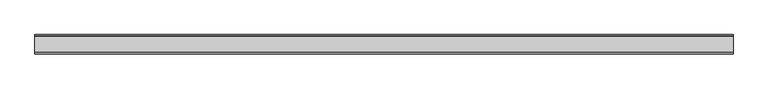
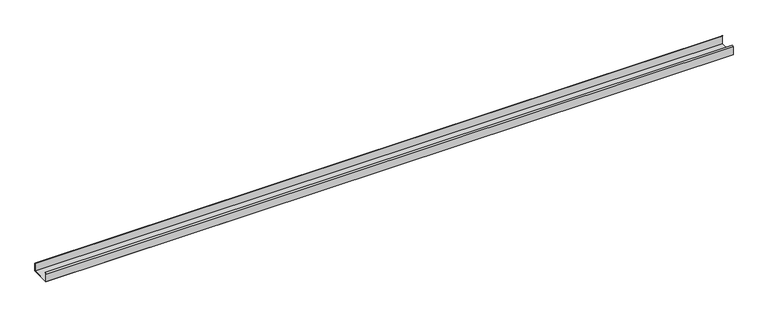
"""IFC4 building model written with IfcOpenShell, lengths in millimetres: proxy geometry, Generic Models 7:Generic Models 1:1:Generic Models 1:1 : Generic Models 7:Generic Models 1:337419:5 : Generic Models 7:Generic Models 1:1:Generic Models 1:1 : Generic Models 7:Generic Models 1:337419:306201."""

from ifc_helpers import new_model, si_unit, frame, origin, place, context, project, spatial, polyline, outline, extrude, source, transform, mapped, element, save


def generic_models_29d2b25b(model_context):
    return source(origin(), model_context, "Body", "SweptSolid", [
        extrude(outline(polyline([(-578797.4913841, 3617.9125), (-579000.6913841, 3617.9125), (-579000.6913841, 3706.8125), (-578986.0982375, 3719.057604), (-578984.3124931, 3716.9294367), (-578997.9132591, 3705.517039), (-578997.9132591, 3620.690625), (-578800.2695091, 3620.690625), (-578800.2695091, 3705.517039), (-578813.8702751, 3716.9294367), (-578812.0845307, 3719.057604), (-578797.4913841, 3706.8125), (-578797.4913841, 3617.9125)])), frame((588867.6367239, 0.0, 0.0), z_axis=(1.0, 0.0, 0.0), x_axis=(0.0, 1.0, 0.0)), (0.0, 0.0, 1.0), 7315.2),
    ])


if __name__ == "__main__":
    model = new_model("IFC4")
    model_context = context("Model", 3, world=origin())
    ifc_project = project(units=[si_unit("LENGTHUNIT", "METRE", prefix="MILLI")], contexts=[model_context])
    site = spatial("IfcSite", under=ifc_project)
    building = spatial("IfcBuilding", under=site)
    placement = place(None, origin())
    generic_models_shape = generic_models_29d2b25b(model_context)
    element("IfcBuildingElementProxy", 1, Name="Generic Models 7:Generic Models 1:1:Generic Models 1:1 : Generic Models 7:Generic Models 1:337419:5 : Generic Models 7:Generic Models 1:1:Generic Models 1:1 : Generic Models 7:Generic Models 1:337419:306201", ObjectType="Generic Models 7:Generic Models 1:1:Generic Models 1:1 : Generic Models 7:Generic Models 1:337419:5 : Generic Models 7:Generic Models 1:1:Generic Models 1:1 : Generic Models 7:Generic Models 1:337419:306201", at=placement, inside=building, context=model_context, shape_type="MappedRepresentation", body=[
        mapped(generic_models_shape, transform((0.0, 0.0, 0.0), x_axis=(1.0, 0.0, 0.0), y_axis=(0.0, 1.0, 0.0), z_axis=(0.0, 0.0, 1.0))),
    ])
    save(model, "model.ifc")

# Revit data of these elements
# Type "Generic Models 7:Generic Models 1:1:Generic Models 1:1 : Generic Models 7:Generic Models 1:337419:5 : Generic Models 7:Generic Models 1:1:Generic Models 1:1 : Generic Models 7:Generic Models 1:337419:306201"
#   NameOverride = "Generic Models 7:Generic Models 1:1:Generic Models 1:1 : Generic Models 7:Generic Models 1:337419:306201"
#   ObjectTypeOverride = "Generic Models 1:1 : Generic Models 7:Generic Models 1:337419"
#   Reference = "Generic Models 1"
#   Tag = "306201"
# Element 1 (IfcBuildingElementProxy, "Generic Models 7:Generic Models 1:1:Generic Models 1:1 : Generic Models 7:Generic Models 1:337419:5 : Generic Models 7:Generic Models 1:1:Generic Models 1:1 : Generic Models 7:Generic Models 1:337419:306201")
#   Materials on its faces: "CEE' SECTION (8.0x3.5C - SEE STRUCT. DWGS)"
# Materials
#   "CEE' SECTION (8.0x3.5C - SEE STRUCT. DWGS)": class "Unassigned", colour RGB 210 209 208, transparency 0, Keynote = "M05121300.02", Cost = 0
